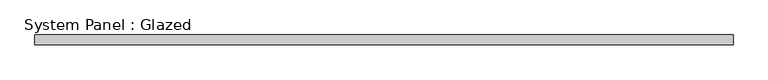
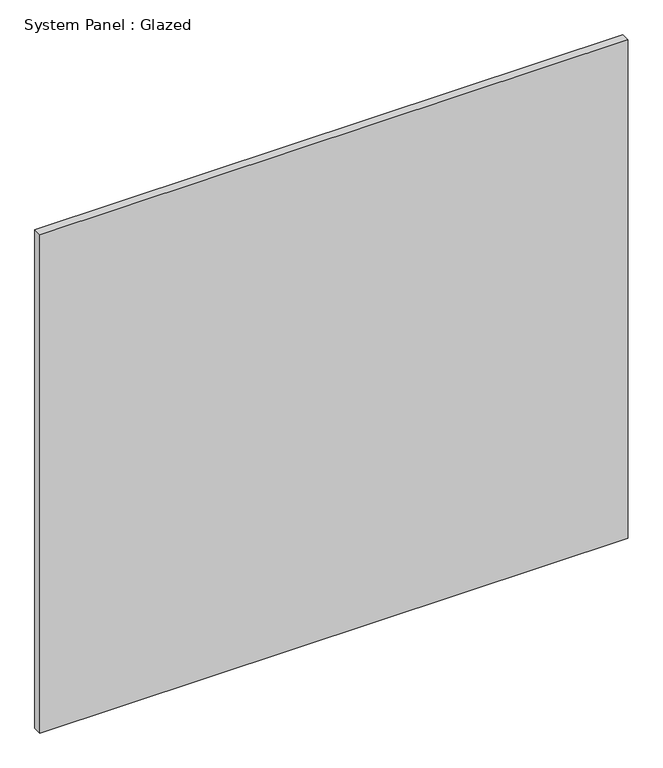
"""IFC4 building model written with IfcOpenShell, lengths in millimetres: plate geometry, System Panel : Glazed."""

import ifcopenshell
import ifcopenshell.guid

model = None  # the IFC model being written
_history = None  # IfcOwnerHistory: only IFC2X3 demands one
_inside = {}  # id of a spatial element -> (the spatial element, [elements in it])
_under = {}  # id of a project, library or spatial element -> (it, [spatial elements below it])
_declared = {}  # id of a project -> (the project, [libraries it declares])
_typed = {}  # id of a type object -> (the type object, [elements of that type])
_made_of = {}  # id of a material, layer set ... -> (it, [elements and type objects made of it])


def new_model(schema):
    """Start an empty IFC model of exactly this schema.

    Asked for "IFC4X3", IfcOpenShell would pick the latest addendum, in which some entities
    have other attributes; the version numbers below select the first issue.
    IFC2X3 requires an IfcOwnerHistory on every rooted entity: one is made here for all.
    """
    global model, _history
    if schema == "IFC4X3":
        model = ifcopenshell.file(schema_version=(4, 3, 0, 0))
    else:
        model = ifcopenshell.file(schema=schema)
    _inside.clear()
    _under.clear()
    _declared.clear()
    _typed.clear()
    _made_of.clear()
    _history = None
    if model.schema == "IFC2X3":
        org = make("IfcOrganization", Name="unknown")
        user = make(
            "IfcPersonAndOrganization",
            ThePerson=make("IfcPerson", FamilyName="unknown"),
            TheOrganization=org,
        )
        app = make(
            "IfcApplication",
            ApplicationDeveloper=org,
            Version="unknown",
            ApplicationFullName="unknown",
            ApplicationIdentifier="unknown",
        )
        _history = make(
            "IfcOwnerHistory",
            OwningUser=user,
            OwningApplication=app,
            ChangeAction="ADDED",
            CreationDate=0,
        )
    return model


def make(cls, **values):
    """One entity of the class cls with the attributes given. An attribute that is None is left unset."""
    return model.create_entity(
        cls, **{name: value for name, value in values.items() if value is not None}
    )


def rooted(cls, **values):
    """An entity with a GlobalId (a new one), such as an element, a storey or a relation."""
    return make(cls, GlobalId=ifcopenshell.guid.new(), OwnerHistory=_history, **values)


def si_unit(unit_type, name, prefix=None):
    """IfcSIUnit, for example si_unit("LENGTHUNIT", "METRE", prefix="MILLI")."""
    return make("IfcSIUnit", UnitType=unit_type, Prefix=prefix, Name=name)


def assignment(units):
    """IfcUnitAssignment: the units of a project."""
    return None if units is None else make("IfcUnitAssignment", Units=units)


def point(xyz):
    """IfcCartesianPoint."""
    return None if xyz is None else make("IfcCartesianPoint", Coordinates=xyz)


def direction(xyz):
    """IfcDirection."""
    return None if xyz is None else make("IfcDirection", DirectionRatios=xyz)


def frame(location, z_axis=None, x_axis=None):
    """IfcAxis2Placement3D, a coordinate frame: its origin and axes. An axis left out is left unset."""
    return make(
        "IfcAxis2Placement3D",
        Location=point(location),
        Axis=direction(z_axis),
        RefDirection=direction(x_axis),
    )


def origin():
    """The frame at (0, 0, 0) with its axes left unset."""
    return frame((0.0, 0.0, 0.0))


def origin_with_axes():
    """The frame at (0, 0, 0) with the z axis (0, 0, 1) and the x axis (1, 0, 0) written out."""
    return frame((0.0, 0.0, 0.0), z_axis=(0.0, 0.0, 1.0), x_axis=(1.0, 0.0, 0.0))


def place(relative_to, where):
    """IfcLocalPlacement: puts the frame where relative to a parent placement (None: the world)."""
    return make(
        "IfcLocalPlacement", PlacementRelTo=relative_to, RelativePlacement=where
    )


def context(
    kind, dimensions, precision=None, world=None, true_north=None, identifier=None
):
    """IfcGeometricRepresentationContext, for example the 3D "Model" context."""
    return make(
        "IfcGeometricRepresentationContext",
        ContextIdentifier=identifier,
        ContextType=kind,
        CoordinateSpaceDimension=dimensions,
        Precision=precision,
        WorldCoordinateSystem=world,
        TrueNorth=true_north,
    )


def project(units=None, contexts=None):
    """IfcProject with its units and contexts."""
    return rooted(
        "IfcProject",
        Name="project",
        RepresentationContexts=contexts,
        UnitsInContext=assignment(units),
    )


def spatial(cls, under=None, at=None, **own):
    """A site, building, storey or space (cls), placed at a placement, below another one or the project."""
    s = rooted(cls, ObjectPlacement=at, **own)
    if under is not None:
        _under.setdefault(under.id(), (under, []))[1].append(s)
    return s


def polyline(points):
    """IfcPolyline through the points."""
    return make("IfcPolyline", Points=[point(p) for p in points])


def outline(outer, holes=None, kind="AREA"):
    """IfcArbitraryClosedProfileDef: a profile drawn as a closed curve; with holes, ...WithVoids."""
    if holes is None:
        return make("IfcArbitraryClosedProfileDef", ProfileType=kind, OuterCurve=outer)
    return make(
        "IfcArbitraryProfileDefWithVoids",
        ProfileType=kind,
        OuterCurve=outer,
        InnerCurves=holes,
    )


def extrude(swept, where, along, depth):
    """IfcExtrudedAreaSolid: the profile swept, set in the frame where, extruded along a direction by depth."""
    return make(
        "IfcExtrudedAreaSolid",
        SweptArea=swept,
        Position=where,
        ExtrudedDirection=direction(along),
        Depth=depth,
    )


def shape(context_of_items, identifier, shape_type, items):
    """IfcShapeRepresentation: the items that make up one representation, for example the "Body"."""
    return make(
        "IfcShapeRepresentation",
        ContextOfItems=context_of_items,
        RepresentationIdentifier=identifier,
        RepresentationType=shape_type,
        Items=items,
    )


def source(mapping_origin, context_of_items, identifier, shape_type, items):
    """IfcRepresentationMap: a shape defined once, which mapped items show again and again."""
    return make(
        "IfcRepresentationMap",
        MappingOrigin=mapping_origin,
        MappedRepresentation=shape(context_of_items, identifier, shape_type, items),
    )


def transform(
    local_origin,
    x_axis=None,
    y_axis=None,
    z_axis=None,
    scale=None,
    scale2=None,
    scale3=None,
    uniform=True,
):
    """IfcCartesianTransformationOperator3D, or its non-uniform kind. x_axis, y_axis, z_axis: its Axis1, 2, 3."""
    if uniform:
        return make(
            "IfcCartesianTransformationOperator3D",
            Axis1=direction(x_axis),
            Axis2=direction(y_axis),
            LocalOrigin=point(local_origin),
            Scale=scale,
            Axis3=direction(z_axis),
        )
    return make(
        "IfcCartesianTransformationOperator3DnonUniform",
        Axis1=direction(x_axis),
        Axis2=direction(y_axis),
        LocalOrigin=point(local_origin),
        Scale=scale,
        Axis3=direction(z_axis),
        Scale2=scale2,
        Scale3=scale3,
    )


def mapped(mapping_source, mapping_target):
    """IfcMappedItem: shows the shape of a source again, moved by a transform."""
    return make(
        "IfcMappedItem", MappingSource=mapping_source, MappingTarget=mapping_target
    )


def made_of(thing, what):
    """Note that an element or type object is made of a material, layer set ...; save() writes the relation."""
    if what is not None:
        _made_of.setdefault(what.id(), (what, []))[1].append(thing)
    return thing


def element(
    cls,
    number,
    at=None,
    inside=None,
    cuts=None,
    type_object=None,
    material=None,
    context=None,
    identifier="Body",
    shape_type=None,
    held_by="IfcProductDefinitionShape",
    body=None,
    shapes=None,
    **own,
):
    """One element of the class cls, such as IfcWall. Its Tag is "e" and its number.

    at: its placement. inside: the storey or other place that contains it. cuts: it is an
    opening in that element (IfcRelVoidsElement). A single representation is given by context,
    identifier, shape_type and body (its items); several are given by shapes. held_by: the class
    of the entity that holds the representations. save() writes the other relations.
    """
    e = rooted(cls, Tag="e%d" % number, ObjectPlacement=at, **own)
    if body is not None:
        shapes = [shape(context, identifier, shape_type, body)]
    if shapes is not None:
        e.Representation = make(held_by, Representations=shapes)
    if inside is not None:
        _inside.setdefault(inside.id(), (inside, []))[1].append(e)
    if cuts is not None:
        rooted(
            "IfcRelVoidsElement", RelatingBuildingElement=cuts, RelatedOpeningElement=e
        )
    if type_object is not None:
        _typed.setdefault(type_object.id(), (type_object, []))[1].append(e)
    return made_of(e, material)


def aggregate(whole, parts):
    """IfcRelAggregates: a whole, such as a stair, and the parts it consists of."""
    return rooted("IfcRelAggregates", RelatingObject=whole, RelatedObjects=parts)


def save(model, path):
    """Write the relations noted so far, then the file.

    IfcRelAggregates (storeys below a building ...), IfcRelContainedInSpatialStructure (elements
    in a storey), IfcRelDefinesByType, IfcRelAssociatesMaterial and IfcRelDeclares: one each for
    every whole, place, type object, material and project.
    """
    for whole, parts in _under.values():
        aggregate(whole, parts)
    for where, things in _inside.values():
        rooted(
            "IfcRelContainedInSpatialStructure",
            RelatedElements=things,
            RelatingStructure=where,
        )
    for kind, things in _typed.values():
        rooted("IfcRelDefinesByType", RelatedObjects=things, RelatingType=kind)
    for what, things in _made_of.values():
        rooted("IfcRelAssociatesMaterial", RelatedObjects=things, RelatingMaterial=what)
    for by, libraries in _declared.values():
        rooted("IfcRelDeclares", RelatingContext=by, RelatedDefinitions=libraries)
    model.write(path)


def system_panel_glazed_df2c046e(model_context):
    return source(origin(), model_context, "Body", "SweptSolid", [
        extrude(outline(polyline([(882.65, 19.05), (-882.65, 19.05), (-882.65, 44.45), (882.65, 44.45), (882.65, 19.05)])), origin_with_axes(), (0.0, 0.0, 1.0), 1581.15),
    ])


if __name__ == "__main__":
    model = new_model("IFC4")
    model_context = context("Model", 3, world=origin())
    ifc_project = project(units=[si_unit("LENGTHUNIT", "METRE", prefix="MILLI")], contexts=[model_context])
    site = spatial("IfcSite", under=ifc_project)
    building = spatial("IfcBuilding", under=site)
    placement = place(None, origin())
    system_panel_glazed_shape = system_panel_glazed_df2c046e(model_context)
    element("IfcPlate", 1, ObjectType="System Panel : Glazed", at=placement, inside=building, context=model_context, shape_type="MappedRepresentation", body=[
        mapped(system_panel_glazed_shape, transform((0.0, 0.0, 0.0), x_axis=(1.0, 0.0, 0.0), y_axis=(0.0, 1.0, 0.0), z_axis=(0.0, 0.0, 1.0))),
    ])
    save(model, "model.ifc")

# Revit data of these elements
# Type "System Panel : Glazed"
#   Construction Type Id = "GSP4R"
#   Analytic Construction = "1/8 in Pilkington single glazing"
#   Visual Light Transmittance = 0.9
#   Solar Heat Gain Coefficient = 0.86
#   Heat Transfer Coefficient (U) = 1.18115 BTU/(h·ft²·°F)
#   Define Thermal Properties by = 1
# Element 1 (IfcPlate, "System Panel : Glazed")
#   Materials on its faces: "Glass"
# Materials
#   "Glass": class "Glass", colour RGB 0 128 192, transparency 0.75, Description = "Soda Lime Glass", Cost = 0
